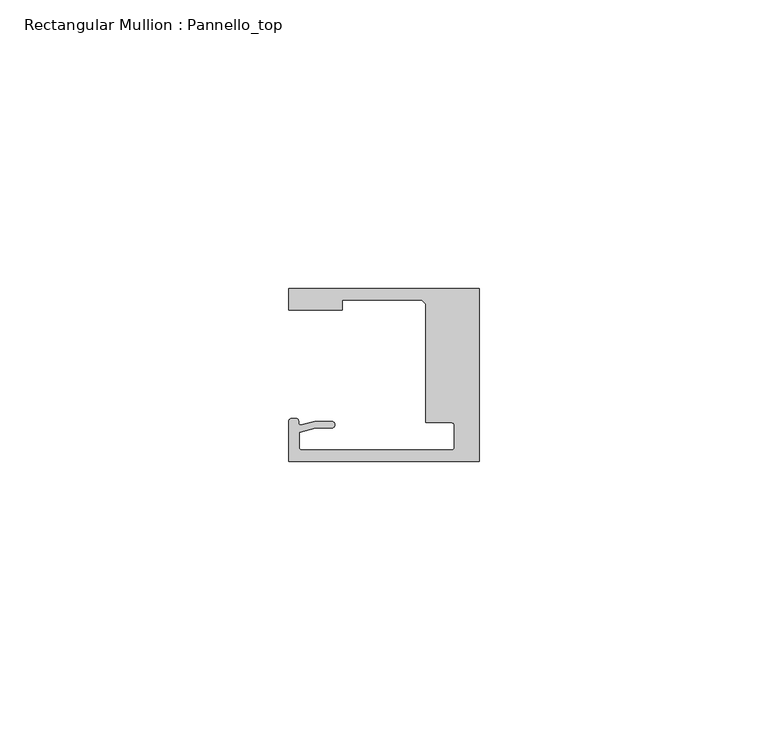
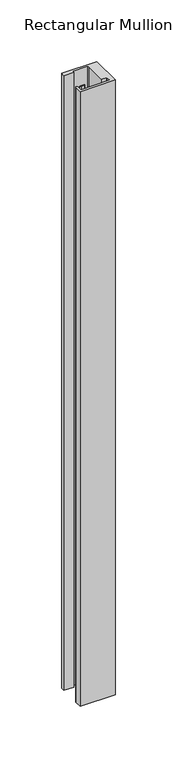
"""IFC4 building model written with IfcOpenShell, lengths in millimetres: member geometry, Rectangular Mullion : Pannello_top."""

from ifc_helpers import new_model, si_unit, frame, origin, place, context, project, spatial, polyline, circle_curve, source, transform, mapped, element, save
from ifc_brep_helpers import plane_surface, cylinder_surface, revolved_surface, extruded_surface, spline_curve, advanced_brep


def rectangular_mullion_pannello_top_d63c9f7e(model_context):
    return source(origin(), model_context, "Body", "AdvancedBrep", [
        advanced_brep(
        [(-33.0, 15.0, 0.0), (-33.0, 11.3000004, 0.0), (-23.700041, 11.3000004, 0.0), (-23.700041, 13.0000004, 0.0), (-10.0000103, 13.0000004, 0.0), (-9.2999726, 12.2999849, 0.0), (-9.2999726, -8.2500595, 0.0), (-4.7999726, -8.2500595, 0.0), (-4.2999726, -8.7500595, 0.0), (-4.2999726, -12.50001, 0.0), (-4.7999726, -13.00001, 0.0), (-30.69998, -13.00001, 0.0), (-31.19998, -12.50001, 0.0), (-31.19998, -9.9657591, 0.0), (-28.3419477, -9.1999523, 0.0), (-25.59998, -9.1999523, 0.0), (-25.59998, -7.9999523, 0.0), (-28.4999305, -7.9999523, 0.0), (-30.9223017, -8.6490241, 0.0), (-33.0000135, -8.0000472, 0.0), (-33.0000135, -15.0, 0.0), (0.0, -15.0, 0.0), (0.0, 15.0, 0.0), (-33.0, 15.0, -609.0245992), (0.0, 15.0, -609.0245992), (0.0, -15.0, -609.0245992), (-33.0000135, -15.0, -609.0245992), (-33.0000135, -8.0000472, -609.0245992), (-30.9223017, -8.6490241, -609.0245992), (-28.4999305, -7.9999523, -609.0245992), (-25.59998, -7.9999523, -609.0245992), (-25.59998, -9.1999523, -609.0245992), (-28.3419477, -9.1999523, -609.0245992), (-31.19998, -9.9657591, -609.0245992), (-31.19998, -12.50001, -609.0245992), (-30.69998, -13.00001, -609.0245992), (-4.7999726, -13.00001, -609.0245992), (-4.2999726, -12.50001, -609.0245992), (-4.2999726, -8.7500595, -609.0245992), (-4.7999726, -8.2500595, -609.0245992), (-9.2999726, -8.2500595, -609.0245992), (-9.2999726, 12.2999849, -609.0245992), (-10.0000103, 13.0000004, -609.0245992), (-23.700041, 13.0000004, -609.0245992), (-23.700041, 11.3000004, -609.0245992), (-33.0, 11.3000004, -609.0245992)],
        [
            (0, 1),
            (1, 2),
            (2, 3),
            (3, 4),
            (4, 5),
            (5, 6),
            (6, 7),
            (7, 8, circle_curve(frame((-4.7999726, -8.7500595, 0.0), z_axis=(0.0, 0.0, -1.0), x_axis=(0.0, 1.0, 0.0)), 0.5)),
            (8, 9),
            (9, 10, circle_curve(frame((-4.7999726, -12.50001, 0.0), z_axis=(0.0, 0.0, -1.0), x_axis=(1.0, 0.0, 0.0)), 0.5)),
            (10, 11),
            (11, 12, circle_curve(frame((-30.69998, -12.50001, 0.0), z_axis=(0.0, 0.0, -1.0), x_axis=(0.0, -1.0, 0.0)), 0.5)),
            (12, 13),
            (13, 14),
            (14, 15),
            (15, 16, circle_curve(frame((-25.59998, -8.5999523, 0.0), z_axis=(0.0, 0.0, 1.0), x_axis=(0.0, -1.0, 0.0)), 0.6)),
            (16, 17),
            (17, 18),
            (18, 19, spline_curve(3, [(-30.9223017, -8.6490241, 0.0), (-31.312054066, -8.717747958, 0.0), (-31.298563602, -8.366228555, 0.0), (-31.305645054, -7.690065204, 0.0), (-31.357433266, -7.563996614, 0.0), (-32.262327879, -7.456527435, 0.0), (-33.0000135, -7.457047519, 0.0), (-33.0000135, -8.0000472, 0.0)], [4, 2, 2, 4], [0.0, 0.001840817752199412, 0.004996616814974408, 0.007702013405570312])),
            (19, 20),
            (20, 21),
            (21, 22),
            (22, 0),
            (23, 24),
            (24, 25),
            (25, 26),
            (26, 27),
            (27, 28, spline_curve(3, [(-33.0000135, -8.0000472, -609.0245992), (-33.0000135, -7.457047519, -609.0245992), (-32.262327879, -7.456527435, -609.0245992), (-31.357433266, -7.563996614, -609.0245992), (-31.305645054, -7.690065204, -609.0245992), (-31.298563602, -8.366228555, -609.0245992), (-31.312054066, -8.717747958, -609.0245992), (-30.9223017, -8.6490241, -609.0245992)], [4, 2, 2, 4], [0.0, 0.0027053965905959043, 0.0058611956533709, 0.007702013405570312])),
            (28, 29),
            (29, 30),
            (30, 31, circle_curve(frame((-25.59998, -8.5999523, -609.0245992), z_axis=(0.0, 0.0, -1.0), x_axis=(0.0, -1.0, 0.0)), 0.6)),
            (31, 32),
            (32, 33),
            (33, 34),
            (34, 35, circle_curve(frame((-30.69998, -12.50001, -609.0245992), z_axis=(0.0, 0.0, 1.0), x_axis=(0.0, -1.0, 0.0)), 0.5)),
            (35, 36),
            (36, 37, circle_curve(frame((-4.7999726, -12.50001, -609.0245992), z_axis=(0.0, 0.0, 1.0), x_axis=(1.0, 0.0, 0.0)), 0.5)),
            (37, 38),
            (38, 39, circle_curve(frame((-4.7999726, -8.7500595, -609.0245992), z_axis=(0.0, 0.0, 1.0), x_axis=(0.0, 1.0, 0.0)), 0.5)),
            (39, 40),
            (40, 41),
            (41, 42),
            (42, 43),
            (43, 44),
            (44, 45),
            (45, 23),
            (0, 23),
            (45, 1),
            (44, 2),
            (43, 3),
            (42, 4),
            (41, 5),
            (40, 6),
            (39, 7),
            (38, 8),
            (37, 9),
            (36, 10),
            (35, 11),
            (34, 12),
            (33, 13),
            (32, 14),
            (31, 15),
            (30, 16),
            (29, 17),
            (28, 18),
            (27, 19),
            (26, 20),
            (25, 21),
            (24, 22),
        ],
        [
            plane_surface(frame((0.0, -36.2491502, 0.0), z_axis=(0.0, 0.0, 1.0), x_axis=(-1.0, 0.0, 0.0))),
            plane_surface(frame((0.0, -36.2491502, -609.0245992), z_axis=(0.0, 0.0, -1.0), x_axis=(-1.0, 0.0, 0.0))),
            plane_surface(frame((-33.0, 15.0, 0.0), z_axis=(-1.0, 0.0, 0.0), x_axis=(0.0, 0.0, -1.0))),
            plane_surface(frame((-33.0, 11.3000004, 0.0), z_axis=(0.0, -1.0, 0.0), x_axis=(0.0, 0.0, -1.0))),
            plane_surface(frame((-23.700041, 11.3000004, 0.0), z_axis=(1.0, 0.0, 0.0), x_axis=(0.0, 0.0, -1.0))),
            plane_surface(frame((-23.700041, 13.0000004, 0.0), z_axis=(0.0, -1.0, 0.0), x_axis=(0.0, 0.0, -1.0))),
            plane_surface(frame((-10.0000103, 13.0000004, 0.0), z_axis=(-0.7070955486277984, -0.7071180135668678, 0.0), x_axis=(0.0, 0.0, -1.0))),
            plane_surface(frame((-9.2999726, 12.2999849, 0.0), z_axis=(-1.0, 0.0, 0.0), x_axis=(0.0, 0.0, -1.0))),
            plane_surface(frame((-9.2999726, -8.2500595, 0.0), z_axis=(0.0, -1.0, 0.0), x_axis=(0.0, 0.0, -1.0))),
            revolved_surface(polyline([(-4.7999726, -8.2500595, -609.0245992), (-4.7999726, -8.2500595, 0.0)]), (-4.7999726, -8.7500595, 0.0), (0.0, 0.0, -1.0)),
            plane_surface(frame((-4.2999726, -8.7500595, 0.0), z_axis=(-1.0, 0.0, 0.0), x_axis=(0.0, 0.0, -1.0))),
            revolved_surface(polyline([(-4.2999726, -12.50001, -609.0245992), (-4.2999726, -12.50001, 0.0)]), (-4.7999726, -12.50001, 0.0), (0.0, 0.0, -1.0)),
            plane_surface(frame((-4.7999726, -13.00001, 0.0), z_axis=(0.0, 1.0, 0.0), x_axis=(0.0, 0.0, -1.0))),
            revolved_surface(polyline([(-30.69998, -13.00001, -609.0245992), (-30.69998, -13.00001, 0.0)]), (-30.69998, -12.50001, 0.0), (0.0, 0.0, -1.0)),
            plane_surface(frame((-31.19998, -12.50001, 0.0), z_axis=(1.0, 0.0, 0.0), x_axis=(0.0, 0.0, -1.0))),
            plane_surface(frame((-31.19998, -9.9657591, 0.0), z_axis=(0.25881883204288636, -0.9659258833782002, 0.0), x_axis=(0.0, 0.0, -1.0))),
            plane_surface(frame((-28.3419477, -9.1999523, 0.0), z_axis=(0.0, -1.0, 0.0), x_axis=(0.0, 0.0, -1.0))),
            cylinder_surface(frame((-25.59998, -8.5999523, 0.0), z_axis=(0.0, 0.0, 1.0), x_axis=(0.0, -1.0, 0.0)), 0.6),
            plane_surface(frame((-25.59998, -7.9999523, 0.0), z_axis=(0.0, 1.0, 0.0), x_axis=(0.0, 0.0, -1.0))),
            plane_surface(frame((-28.4999305, -7.9999523, 0.0), z_axis=(-0.25881883200192934, 0.9659258833891746, 0.0), x_axis=(0.0, 0.0, -1.0))),
            extruded_surface(spline_curve(3, [(-30.9223017, -8.6490241, -609.0245992), (-31.312054066, -8.717747958, -609.0245992), (-31.298563602, -8.366228555, -609.0245992), (-31.305645054, -7.690065204, -609.0245992), (-31.357433266, -7.563996614, -609.0245992), (-32.262327879, -7.456527435, -609.0245992), (-33.0000135, -7.457047519, -609.0245992), (-33.0000135, -8.0000472, -609.0245992)], [4, 2, 2, 4], [0.0, 0.001840817752199412, 0.004996616814974408, 0.007702013405570312]), (0.0, 0.0, 609.0245992), 609.0245992),
            plane_surface(frame((-33.0000135, -8.0000472, 0.0), z_axis=(-1.0, 0.0, 0.0), x_axis=(0.0, 0.0, -1.0))),
            plane_surface(frame((-33.0000135, -15.0, 0.0), z_axis=(0.0, -1.0, 0.0), x_axis=(0.0, 0.0, -1.0))),
            plane_surface(frame((0.0, -15.0, 0.0), z_axis=(1.0, 0.0, 0.0), x_axis=(0.0, 0.0, -1.0))),
            plane_surface(frame((0.0, 15.0, 0.0), z_axis=(0.0, 1.0, 0.0), x_axis=(0.0, 0.0, -1.0))),
        ],
        [
            (0, [[1, 2, 3, 4, 5, 6, 7, 8, 9, 10, 11, 12, 13, 14, 15, 16, 17, 18, 19, 20, 21, 22, 23]]),
            (1, [[24, 25, 26, 27, 28, 29, 30, 31, 32, 33, 34, 35, 36, 37, 38, 39, 40, 41, 42, 43, 44, 45, 46]]),
            (2, [[-1, 47, -46, 48]]),
            (3, [[-2, -48, -45, 49]]),
            (4, [[-3, -49, -44, 50]]),
            (5, [[-4, -50, -43, 51]]),
            (6, [[-5, -51, -42, 52]]),
            (7, [[-6, -52, -41, 53]]),
            (8, [[-7, -53, -40, 54]]),
            (9, [[-8, -54, -39, 55]]),
            (10, [[-9, -55, -38, 56]]),
            (11, [[-10, -56, -37, 57]]),
            (12, [[-11, -57, -36, 58]]),
            (13, [[-12, -58, -35, 59]]),
            (14, [[-13, -59, -34, 60]]),
            (15, [[-14, -60, -33, 61]]),
            (16, [[-15, -61, -32, 62]]),
            (17, [[-16, -62, -31, 63]]),
            (18, [[-17, -63, -30, 64]]),
            (19, [[-18, -64, -29, 65]]),
            (20, [[-19, -65, -28, 66]]),
            (21, [[-20, -66, -27, 67]]),
            (22, [[-21, -67, -26, 68]]),
            (23, [[-22, -68, -25, 69]]),
            (24, [[-23, -69, -24, -47]]),
        ],
    ),
    ])


if __name__ == "__main__":
    model = new_model("IFC4")
    model_context = context("Model", 3, world=origin())
    ifc_project = project(units=[si_unit("LENGTHUNIT", "METRE", prefix="MILLI")], contexts=[model_context])
    site = spatial("IfcSite", under=ifc_project)
    building = spatial("IfcBuilding", under=site)
    placement = place(None, origin())
    rectangular_mullion_pannello_top_shape = rectangular_mullion_pannello_top_d63c9f7e(model_context)
    element("IfcMember", 1, ObjectType="Rectangular Mullion : Pannello_top", at=placement, inside=building, context=model_context, shape_type="MappedRepresentation", body=[
        mapped(rectangular_mullion_pannello_top_shape, transform((0.0, 0.0, 0.0), x_axis=(1.0, 0.0, 0.0), y_axis=(0.0, 1.0, 0.0), z_axis=(0.0, 0.0, 1.0))),
    ])
    save(model, "model.ifc")

# Revit data of these elements
# Type "Rectangular Mullion : Pannello_top"
#   built-in parameter 1007322 = 0.0984252 (stored number, unit not read)
#   built-in parameter 1007321 = 0 (stored number, unit not read)
#   built-in parameter 1007320 = 0.0305117 (stored number, unit not read)
